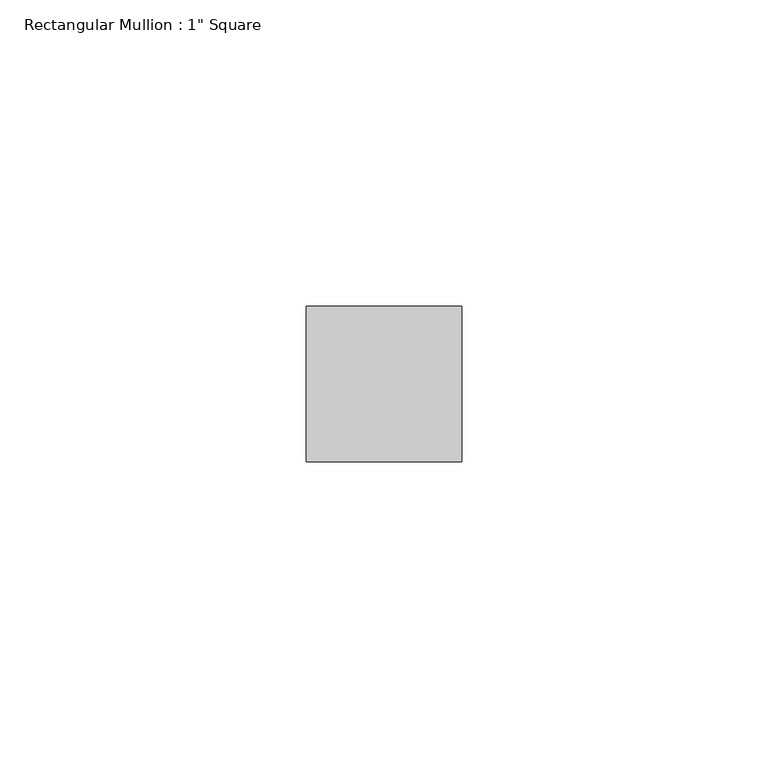
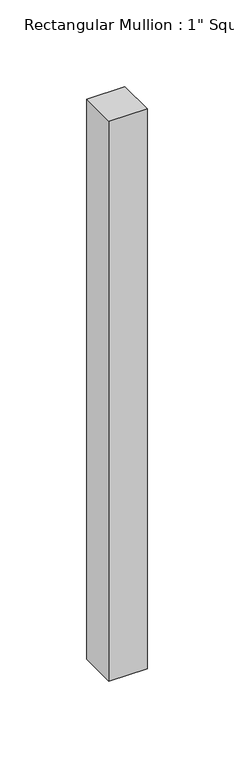
"""IFC4 building model written with IfcOpenShell, lengths in millimetres: member geometry."""

from ifc_helpers import new_model, si_unit, frame, origin, place, context, project, spatial, polyline, outline, extrude, source, transform, mapped, element, save


def member_b53ffca9(model_context):
    return source(origin(), model_context, "Body", "SweptSolid", [
        extrude(outline(polyline([(0.0, 12.7), (0.0, -12.7), (-25.4, -12.7), (-25.4, 12.7), (0.0, 12.7)])), frame((0.0, 0.0, -393.7), z_axis=(0.0, 0.0, 1.0), x_axis=(1.0, 0.0, 0.0)), (0.0, 0.0, 1.0), 393.7),
    ])


if __name__ == "__main__":
    model = new_model("IFC4")
    model_context = context("Model", 3, world=origin())
    ifc_project = project(units=[si_unit("LENGTHUNIT", "METRE", prefix="MILLI")], contexts=[model_context])
    site = spatial("IfcSite", under=ifc_project)
    building = spatial("IfcBuilding", under=site)
    placement = place(None, origin())
    member_shape = member_b53ffca9(model_context)
    element("IfcMember", 1, ObjectType="Rectangular Mullion : 1\" Square", at=placement, inside=building, context=model_context, shape_type="MappedRepresentation", body=[
        mapped(member_shape, transform((0.0, 0.0, 0.0), x_axis=(1.0, 0.0, 0.0), y_axis=(0.0, 1.0, 0.0), z_axis=(0.0, 0.0, 1.0))),
    ])
    save(model, "model.ifc")

# Revit data of these elements
# Type "Rectangular Mullion : 1\" Square"
#   built-in parameter 1007304 = 0.0833333 (stored number, unit not read)
#   built-in parameter 1007301 = 0.0416667 (stored number, unit not read)
#   built-in parameter 1007300 = 0.0416667 (stored number, unit not read)
# Element 1 (IfcMember, "Rectangular Mullion : 1\" Square")
#   Materials on its faces: "Metal - Aluminum"
# Materials
#   "Metal - Aluminum": class "Metal", colour RGB 247 247 247, transparency 0
